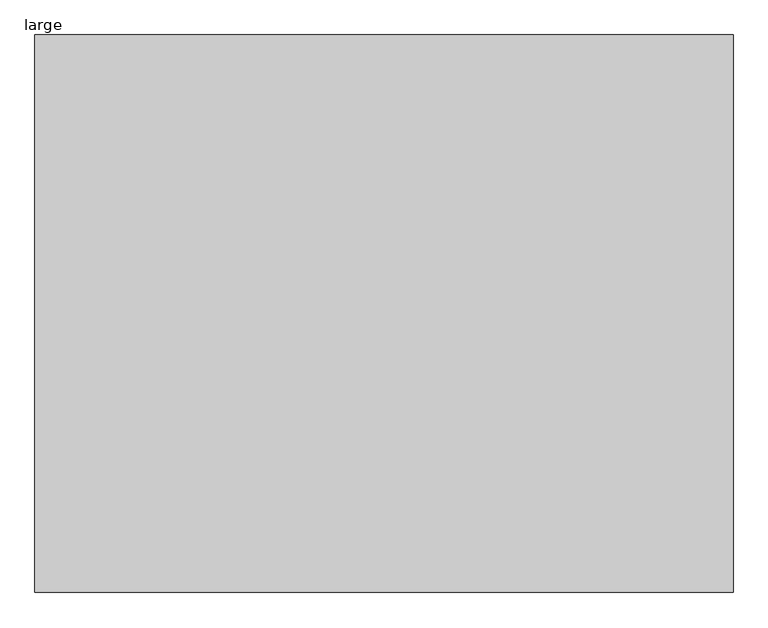
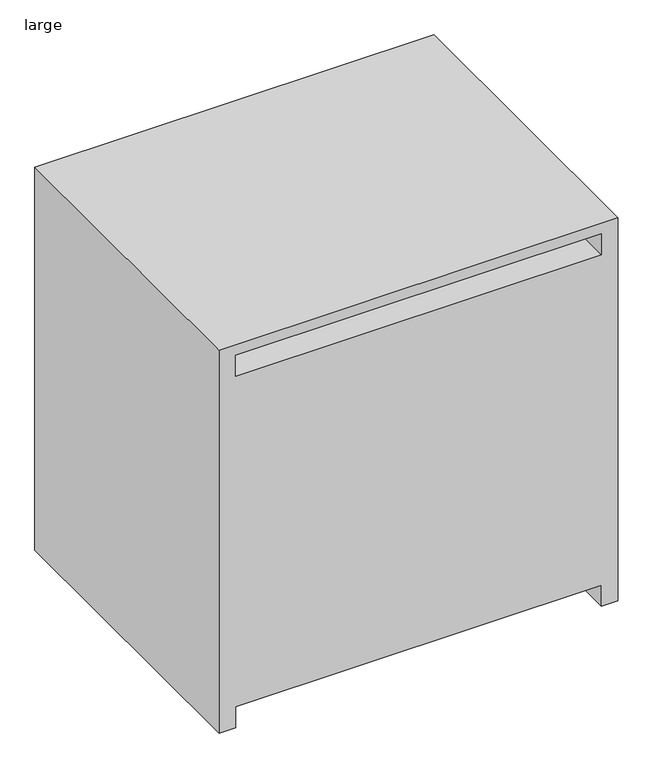
"""IFC4 building model written with IfcOpenShell, lengths in millimetres: proxy geometry, Transformer-Dry-Type-Siemens : large."""

from ifc_helpers import new_model, si_unit, frame, origin, place, context, project, spatial, polyline, outline, extrude, source, transform, mapped, element, save


def large_8446dd82(model_context):
    return source(origin(), model_context, "Body", "SweptSolid", [
        extrude(outline(polyline([(1854.2, 914.4), (1854.2, -914.4), (0.0, -914.4), (0.0, -838.2), (101.6, -838.2), (101.6, 838.2), (0.0, 838.2), (0.0, 914.4), (1854.2, 914.4)]), holes=[polyline([(1803.4, 838.2), (1701.8, 838.2), (1701.8, -838.2), (1803.4, -838.2), (1803.4, 838.2)])]), frame((0.0, -730.25, 0.0), z_axis=(0.0, 1.0, 0.0), x_axis=(0.0, 0.0, 1.0)), (0.0, 0.0, 1.0), 1460.5),
    ])


if __name__ == "__main__":
    model = new_model("IFC4")
    model_context = context("Model", 3, world=origin())
    ifc_project = project(units=[si_unit("LENGTHUNIT", "METRE", prefix="MILLI")], contexts=[model_context])
    site = spatial("IfcSite", under=ifc_project)
    building = spatial("IfcBuilding", under=site)
    placement = place(None, origin())
    large_shape = large_8446dd82(model_context)
    element("IfcBuildingElementProxy", 1, Name="Transformer-Dry-Type-Siemens : large", ObjectType="Transformer-Dry-Type-Siemens : large", at=placement, inside=building, context=model_context, shape_type="MappedRepresentation", body=[
        mapped(large_shape, transform((0.0, 0.0, 0.0), x_axis=(1.0, 0.0, 0.0), y_axis=(0.0, 1.0, 0.0), z_axis=(0.0, 0.0, 1.0))),
    ])
    save(model, "model.ifc")

# Revit data of these elements
# Type "Transformer-Dry-Type-Siemens : large"
#   Weight = "5500"
#   Wattage = "DO NOT USE"
#   Voltage = "DO NOT USE"
#   URL = "http://www.usa.siemens.com/ce"
#   Transformer Material = "Aluminum"
#   Product Page URL = "http://www.sea.siemens.com/us/Products/PowerDistribution/Product/Transformers/Pages/Transformers.aspx"
#   Product Documentation Link = "http://www.sea.siemens.com/us/internet-dms/Internet/ConsultingEngineersComm/General/Docs/drytrans.pdf"
#   Model = "3F3Y015K13TP1"
#   Manufacturer = "Siemens Industry"
#   KVA = "750"
#   K Factor = "13"
#   Description = "Transformer"
#   Deg Rise = "150"
#   Copyright © = "© Siemens Industry, Inc. 2011"
#   CTRL Connector Description = "Equipment Power"
#   BOM URL [instance default] = ""
#   Assembly Code = "D5090900"
#   clearance = 3' - 0"
#   Width = 6' - 0"
#   Primary Voltage = 480 V
#   Power Factor = 1
#   Height = 6' - 1"
#   Depth = 4' - 9 1/2"
#   Apparent Load [instance default] = 0 VA
#   Has Not Contacted Siemens For Configuration [instance default] = no
#   Contacted Siemens For Configuration [instance default] = yes
#   Text Material = Paint- Siemens - Dark
#   Frame Material = ELECTRICAL TRANSFORMERS
# Element 1 (IfcBuildingElementProxy, "Transformer-Dry-Type-Siemens : large")
#   Materials on its faces: "ELECTRICAL TRANSFORMERS"
# Materials
#   "Paint- Siemens - Dark": class "Metal", colour RGB 175 38 68, transparency 0
#   "ELECTRICAL TRANSFORMERS": class "Metal", colour RGB 63 114 97, transparency 0, Cost = 0
